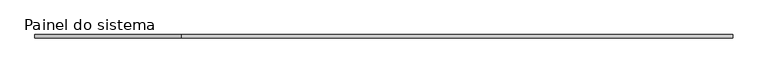
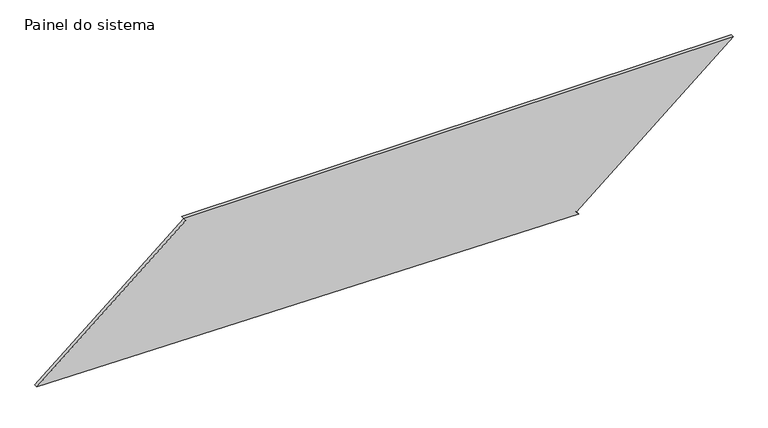
"""IFC4 building model written with IfcOpenShell, lengths in millimetres: plate geometry, Painel do sistema : Envidraçado."""

from ifc_helpers import new_model, si_unit, frame, origin, place, context, project, spatial, polyline, outline, extrude, source, transform, mapped, element, save


def painel_do_sistema_c5ac99e0(model_context):
    return source(origin(), model_context, "Body", "SweptSolid", [
        extrude(outline(polyline([(0.0, 1402.2207254), (19.2037959, 1386.2140323), (964.4326076, 2520.2384741), (964.4326076, -1458.7672557), (945.2288117, -1442.7605627), (47.1325024, -2520.2384741), (0.0, 1402.2207254)])), frame((0.0, 24.5, 0.0), z_axis=(0.0, 1.0, 0.0), x_axis=(0.0, 0.0, 1.0)), (0.0, 0.0, 1.0), 25.0),
    ])


if __name__ == "__main__":
    model = new_model("IFC4")
    model_context = context("Model", 3, world=origin())
    ifc_project = project(units=[si_unit("LENGTHUNIT", "METRE", prefix="MILLI")], contexts=[model_context])
    site = spatial("IfcSite", under=ifc_project)
    building = spatial("IfcBuilding", under=site)
    placement = place(None, origin())
    painel_do_sistema_shape = painel_do_sistema_c5ac99e0(model_context)
    element("IfcPlate", 1, ObjectType="Painel do sistema : Envidraçado", at=placement, inside=building, context=model_context, shape_type="MappedRepresentation", body=[
        mapped(painel_do_sistema_shape, transform((0.0, 0.0, 0.0), x_axis=(1.0, 0.0, 0.0), y_axis=(0.0, 1.0, 0.0), z_axis=(0.0, 0.0, 1.0))),
    ])
    save(model, "model.ifc")

# Revit data of these elements
# Type "Painel do sistema : Envidraçado"
#   Construction Type Id = "GSP4R"
#   Analytic Construction = "Vidraça única Pilkington 1/8 pol"
#   Visual Light Transmittance = 0.9
#   Solar Heat Gain Coefficient = 0.86
#   Heat Transfer Coefficient (U) = 6.7069 W/(m²·K)
# Element 1 (IfcPlate, "Painel do sistema : Envidraçado")
#   Materials on its faces: "Vidro"
# Materials
#   "Vidro": class "Vidro", colour RGB 0 128 192, transparency 0.9, Description = "Vidro de sílica", Cost = 0
